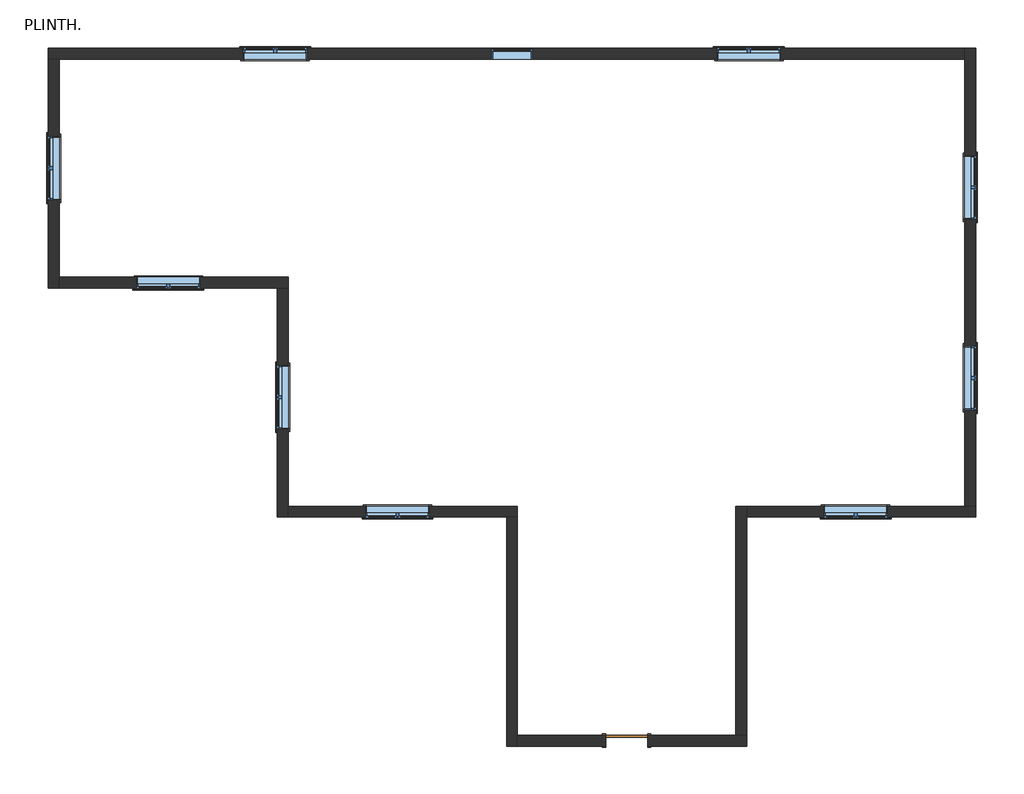
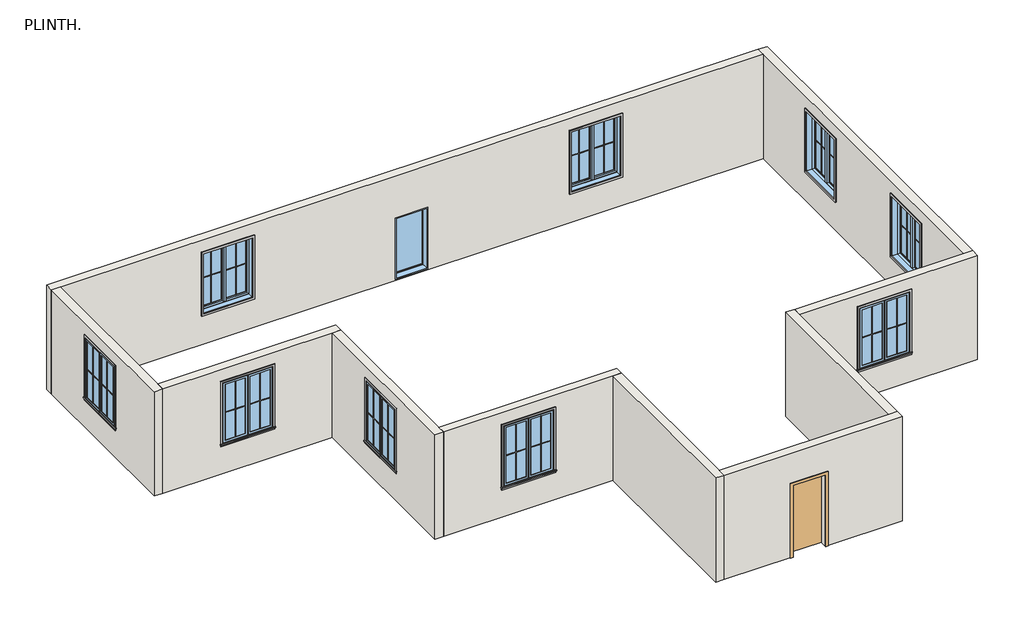
# One storey: 36 proxies, 10 walls, 10 windows, 1 door.
"""IFC4 building model written with IfcOpenShell, lengths in millimetres."""

import ifcopenshell
import ifcopenshell.guid

model = None  # the IFC model being written
_history = None  # IfcOwnerHistory: only IFC2X3 demands one
_inside = {}  # id of a spatial element -> (the spatial element, [elements in it])
_under = {}  # id of a project, library or spatial element -> (it, [spatial elements below it])
_declared = {}  # id of a project -> (the project, [libraries it declares])
_typed = {}  # id of a type object -> (the type object, [elements of that type])
_made_of = {}  # id of a material, layer set ... -> (it, [elements and type objects made of it])


def new_model(schema):
    """Start an empty IFC model of exactly this schema.

    Asked for "IFC4X3", IfcOpenShell would pick the latest addendum, in which some entities
    have other attributes; the version numbers below select the first issue.
    IFC2X3 requires an IfcOwnerHistory on every rooted entity: one is made here for all.
    """
    global model, _history
    if schema == "IFC4X3":
        model = ifcopenshell.file(schema_version=(4, 3, 0, 0))
    else:
        model = ifcopenshell.file(schema=schema)
    _inside.clear()
    _under.clear()
    _declared.clear()
    _typed.clear()
    _made_of.clear()
    _history = None
    if model.schema == "IFC2X3":
        org = make("IfcOrganization", Name="unknown")
        user = make(
            "IfcPersonAndOrganization",
            ThePerson=make("IfcPerson", FamilyName="unknown"),
            TheOrganization=org,
        )
        app = make(
            "IfcApplication",
            ApplicationDeveloper=org,
            Version="unknown",
            ApplicationFullName="unknown",
            ApplicationIdentifier="unknown",
        )
        _history = make(
            "IfcOwnerHistory",
            OwningUser=user,
            OwningApplication=app,
            ChangeAction="ADDED",
            CreationDate=0,
        )
    return model


def make(cls, **values):
    """One entity of the class cls with the attributes given. An attribute that is None is left unset."""
    return model.create_entity(
        cls, **{name: value for name, value in values.items() if value is not None}
    )


def rooted(cls, **values):
    """An entity with a GlobalId (a new one), such as an element, a storey or a relation."""
    return make(cls, GlobalId=ifcopenshell.guid.new(), OwnerHistory=_history, **values)


def si_unit(unit_type, name, prefix=None):
    """IfcSIUnit, for example si_unit("LENGTHUNIT", "METRE", prefix="MILLI")."""
    return make("IfcSIUnit", UnitType=unit_type, Prefix=prefix, Name=name)


def assignment(units):
    """IfcUnitAssignment: the units of a project."""
    return None if units is None else make("IfcUnitAssignment", Units=units)


def point(xyz):
    """IfcCartesianPoint."""
    return None if xyz is None else make("IfcCartesianPoint", Coordinates=xyz)


def direction(xyz):
    """IfcDirection."""
    return None if xyz is None else make("IfcDirection", DirectionRatios=xyz)


def frame(location, z_axis=None, x_axis=None):
    """IfcAxis2Placement3D, a coordinate frame: its origin and axes. An axis left out is left unset."""
    return make(
        "IfcAxis2Placement3D",
        Location=point(location),
        Axis=direction(z_axis),
        RefDirection=direction(x_axis),
    )


def origin():
    """The frame at (0, 0, 0) with its axes left unset."""
    return frame((0.0, 0.0, 0.0))


def origin_with_axes():
    """The frame at (0, 0, 0) with the z axis (0, 0, 1) and the x axis (1, 0, 0) written out."""
    return frame((0.0, 0.0, 0.0), z_axis=(0.0, 0.0, 1.0), x_axis=(1.0, 0.0, 0.0))


def place(relative_to, where):
    """IfcLocalPlacement: puts the frame where relative to a parent placement (None: the world)."""
    return make(
        "IfcLocalPlacement", PlacementRelTo=relative_to, RelativePlacement=where
    )


def context(
    kind, dimensions, precision=None, world=None, true_north=None, identifier=None
):
    """IfcGeometricRepresentationContext, for example the 3D "Model" context."""
    return make(
        "IfcGeometricRepresentationContext",
        ContextIdentifier=identifier,
        ContextType=kind,
        CoordinateSpaceDimension=dimensions,
        Precision=precision,
        WorldCoordinateSystem=world,
        TrueNorth=true_north,
    )


def project(units=None, contexts=None):
    """IfcProject with its units and contexts."""
    return rooted(
        "IfcProject",
        Name="project",
        RepresentationContexts=contexts,
        UnitsInContext=assignment(units),
    )


def spatial(cls, under=None, at=None, **own):
    """A site, building, storey or space (cls), placed at a placement, below another one or the project."""
    s = rooted(cls, ObjectPlacement=at, **own)
    if under is not None:
        _under.setdefault(under.id(), (under, []))[1].append(s)
    return s


def polyline(points):
    """IfcPolyline through the points."""
    return make("IfcPolyline", Points=[point(p) for p in points])


def outline(outer, holes=None, kind="AREA"):
    """IfcArbitraryClosedProfileDef: a profile drawn as a closed curve; with holes, ...WithVoids."""
    if holes is None:
        return make("IfcArbitraryClosedProfileDef", ProfileType=kind, OuterCurve=outer)
    return make(
        "IfcArbitraryProfileDefWithVoids",
        ProfileType=kind,
        OuterCurve=outer,
        InnerCurves=holes,
    )


def extrude(swept, where, along, depth):
    """IfcExtrudedAreaSolid: the profile swept, set in the frame where, extruded along a direction by depth."""
    return make(
        "IfcExtrudedAreaSolid",
        SweptArea=swept,
        Position=where,
        ExtrudedDirection=direction(along),
        Depth=depth,
    )


def faces_of(points, faces, orient=None, outer=None):
    """IfcFace entities. A face is a list of loops; a loop is a list of indices into points, from 0.

    orient and outer hold one flag for each loop. By default every Orientation is true, the
    first loop of a face is its IfcFaceOuterBound and the others are IfcFaceBound.
    """
    made = []
    for i, loops in enumerate(faces):
        bounds = []
        for j, loop in enumerate(loops):
            is_outer = j == 0 if outer is None else outer[i][j]
            bounds.append(
                make(
                    "IfcFaceOuterBound" if is_outer else "IfcFaceBound",
                    Bound=make("IfcPolyLoop", Polygon=[points[k] for k in loop]),
                    Orientation=True if orient is None else orient[i][j],
                )
            )
        made.append(make("IfcFace", Bounds=bounds))
    return made


def faceted_brep(points, faces, orient=None, outer=None, voids=None):
    """IfcFacetedBrep: a solid bounded by flat faces; with voids (closed shells), ...WithVoids."""
    shared = [point(p) for p in points]
    hull = make("IfcClosedShell", CfsFaces=faces_of(shared, faces, orient, outer))
    if voids is None:
        return make("IfcFacetedBrep", Outer=hull)
    return make(
        "IfcFacetedBrepWithVoids",
        Outer=hull,
        Voids=[
            make(cls, CfsFaces=faces_of(shared, fs, o, b)) for cls, fs, o, b in voids
        ],
    )


def shape(context_of_items, identifier, shape_type, items):
    """IfcShapeRepresentation: the items that make up one representation, for example the "Body"."""
    return make(
        "IfcShapeRepresentation",
        ContextOfItems=context_of_items,
        RepresentationIdentifier=identifier,
        RepresentationType=shape_type,
        Items=items,
    )


def source(mapping_origin, context_of_items, identifier, shape_type, items):
    """IfcRepresentationMap: a shape defined once, which mapped items show again and again."""
    return make(
        "IfcRepresentationMap",
        MappingOrigin=mapping_origin,
        MappedRepresentation=shape(context_of_items, identifier, shape_type, items),
    )


def transform(
    local_origin,
    x_axis=None,
    y_axis=None,
    z_axis=None,
    scale=None,
    scale2=None,
    scale3=None,
    uniform=True,
):
    """IfcCartesianTransformationOperator3D, or its non-uniform kind. x_axis, y_axis, z_axis: its Axis1, 2, 3."""
    if uniform:
        return make(
            "IfcCartesianTransformationOperator3D",
            Axis1=direction(x_axis),
            Axis2=direction(y_axis),
            LocalOrigin=point(local_origin),
            Scale=scale,
            Axis3=direction(z_axis),
        )
    return make(
        "IfcCartesianTransformationOperator3DnonUniform",
        Axis1=direction(x_axis),
        Axis2=direction(y_axis),
        LocalOrigin=point(local_origin),
        Scale=scale,
        Axis3=direction(z_axis),
        Scale2=scale2,
        Scale3=scale3,
    )


def mapped(mapping_source, mapping_target):
    """IfcMappedItem: shows the shape of a source again, moved by a transform."""
    return make(
        "IfcMappedItem", MappingSource=mapping_source, MappingTarget=mapping_target
    )


def made_of(thing, what):
    """Note that an element or type object is made of a material, layer set ...; save() writes the relation."""
    if what is not None:
        _made_of.setdefault(what.id(), (what, []))[1].append(thing)
    return thing


def element(
    cls,
    number,
    at=None,
    inside=None,
    cuts=None,
    type_object=None,
    material=None,
    context=None,
    identifier="Body",
    shape_type=None,
    held_by="IfcProductDefinitionShape",
    body=None,
    shapes=None,
    **own,
):
    """One element of the class cls, such as IfcWall. Its Tag is "e" and its number.

    at: its placement. inside: the storey or other place that contains it. cuts: it is an
    opening in that element (IfcRelVoidsElement). A single representation is given by context,
    identifier, shape_type and body (its items); several are given by shapes. held_by: the class
    of the entity that holds the representations. save() writes the other relations.
    """
    e = rooted(cls, Tag="e%d" % number, ObjectPlacement=at, **own)
    if body is not None:
        shapes = [shape(context, identifier, shape_type, body)]
    if shapes is not None:
        e.Representation = make(held_by, Representations=shapes)
    if inside is not None:
        _inside.setdefault(inside.id(), (inside, []))[1].append(e)
    if cuts is not None:
        rooted(
            "IfcRelVoidsElement", RelatingBuildingElement=cuts, RelatedOpeningElement=e
        )
    if type_object is not None:
        _typed.setdefault(type_object.id(), (type_object, []))[1].append(e)
    return made_of(e, material)


def aggregate(whole, parts):
    """IfcRelAggregates: a whole, such as a stair, and the parts it consists of."""
    return rooted("IfcRelAggregates", RelatingObject=whole, RelatedObjects=parts)


def save(model, path):
    """Write the relations noted so far, then the file.

    IfcRelAggregates (storeys below a building ...), IfcRelContainedInSpatialStructure (elements
    in a storey), IfcRelDefinesByType, IfcRelAssociatesMaterial and IfcRelDeclares: one each for
    every whole, place, type object, material and project.
    """
    for whole, parts in _under.values():
        aggregate(whole, parts)
    for where, things in _inside.values():
        rooted(
            "IfcRelContainedInSpatialStructure",
            RelatedElements=things,
            RelatingStructure=where,
        )
    for kind, things in _typed.values():
        rooted("IfcRelDefinesByType", RelatedObjects=things, RelatingType=kind)
    for what, things in _made_of.values():
        rooted("IfcRelAssociatesMaterial", RelatedObjects=things, RelatingMaterial=what)
    for by, libraries in _declared.values():
        rooted("IfcRelDeclares", RelatingContext=by, RelatedDefinitions=libraries)
    model.write(path)


def m_muntin_pattern_2x2_m_muntin_pattern_2x2_d2d4b859(model_context):
    return source(origin(), model_context, "Body", "SweptSolid", [
        extrude(outline(polyline([(836.5, -6.35), (836.5, -281.7375), (823.8, -281.7375), (823.8, -6.35), (0.0, -6.35), (0.0, 6.35), (823.8, 6.35), (823.8, 281.7375), (836.5, 281.7375), (836.5, 6.35), (1660.3, 6.35), (1660.3, -6.35), (836.5, -6.35)])), frame((0.0, 9.525, 0.0), z_axis=(0.0, 1.0, 0.0), x_axis=(0.0, 0.0, 1.0)), (0.0, 0.0, 1.0), 12.7),
        extrude(outline(polyline([(836.5, -6.35), (836.5, -281.7375), (823.8, -281.7375), (823.8, -6.35), (0.0, -6.35), (0.0, 6.35), (823.8, 6.35), (823.8, 281.7375), (836.5, 281.7375), (836.5, 6.35), (1660.3, 6.35), (1660.3, -6.35), (836.5, -6.35)])), frame((0.0, -22.225, 0.0), z_axis=(0.0, 1.0, 0.0), x_axis=(0.0, 0.0, 1.0)), (0.0, 0.0, 1.0), 12.7),
    ])


def m_muntin_pattern_2x2_m_muntin_pattern_2x2_f3921bb5(model_context):
    return source(origin(), model_context, "Body", "SweptSolid", [
        extrude(outline(polyline([(836.5, -6.35), (836.5, -281.7375), (823.8, -281.7375), (823.8, -6.35), (0.0, -6.35), (0.0, 6.35), (823.8, 6.35), (823.8, 281.7375), (836.5, 281.7375), (836.5, 6.35), (1660.3, 6.35), (1660.3, -6.35), (836.5, -6.35)])), frame((0.0, -22.225, 0.0), z_axis=(0.0, 1.0, 0.0), x_axis=(0.0, 0.0, 1.0)), (0.0, 0.0, 1.0), 12.7),
        extrude(outline(polyline([(836.5, -6.35), (836.5, -281.7375), (823.8, -281.7375), (823.8, -6.35), (0.0, -6.35), (0.0, 6.35), (823.8, 6.35), (823.8, 281.7375), (836.5, 281.7375), (836.5, 6.35), (1660.3, 6.35), (1660.3, -6.35), (836.5, -6.35)])), frame((0.0, 9.525, 0.0), z_axis=(0.0, 1.0, 0.0), x_axis=(0.0, 0.0, 1.0)), (0.0, 0.0, 1.0), 12.7),
    ])


def m_trim_window_exterior_flat_with_sill_136e302d(model_context):
    return source(origin(), model_context, "Body", "SweptSolid", [
        extrude(outline(polyline([(760.0, -1820.4323709), (760.0, -1880.4323709), (-760.0, -1880.4323709), (-760.0, -1820.4323709), (760.0, -1820.4323709)])), origin_with_axes(), (0.0, 0.0, 1.0), 19.05),
        extrude(outline(polyline([(-1830.0, 38.1), (-1802.4580645, 38.1), (-1800.0, 19.05), (-1800.0, 0.0), (-1820.4323709, 0.0), (-1820.4323709, 19.05), (-1830.0, 19.05), (-1830.0, 38.1)])), frame((-772.7, 0.0, 0.0), z_axis=(1.0, 0.0, 0.0), x_axis=(0.0, 1.0, 0.0)), (0.0, 0.0, 1.0), 1545.4),
        extrude(outline(polyline([(-760.0, 60.0), (760.0, 60.0), (760.0, -1800.0), (700.0, -1800.0), (700.0, 0.0), (-700.0, 0.0), (-700.0, -1800.0), (-760.0, -1800.0), (-760.0, 60.0)])), origin_with_axes(), (0.0, 0.0, 1.0), 19.05),
    ])


def m_trim_window_interior_flat_picture_frame_c6c50358(model_context):
    return source(origin(), model_context, "Body", "SweptSolid", [
        extrude(outline(polyline([(747.3, 47.3), (747.3, -1847.3), (-747.3, -1847.3), (-747.3, 47.3), (747.3, 47.3)]), holes=[polyline([(687.3, -12.7), (-687.3, -12.7), (-687.3, -1787.3), (687.3, -1787.3), (687.3, -12.7)])]), origin_with_axes(), (0.0, 0.0, 1.0), 30.0),
    ])


def m_single_flush_0915_x_2134mm_c020cfaa(model_context):
    return source(origin(), model_context, "Body", "SweptSolid", [
        extrude(outline(polyline([(2210.0, -533.5), (0.0, -533.5), (0.0, -457.5), (2134.0, -457.5), (2134.0, 457.5), (0.0, 457.5), (0.0, 533.5), (2210.0, 533.5), (2210.0, -533.5)])), frame((0.0, 120.0, 0.0), z_axis=(0.0, 1.0, 0.0), x_axis=(0.0, 0.0, 1.0)), (0.0, 0.0, 1.0), 25.0),
        extrude(outline(polyline([(2210.0, 533.5), (2210.0, -533.5), (0.0, -533.5), (0.0, -457.5), (2134.0, -457.5), (2134.0, 457.5), (0.0, 457.5), (0.0, 533.5), (2210.0, 533.5)])), frame((0.0, -145.0, 0.0), z_axis=(0.0, 1.0, 0.0), x_axis=(0.0, 0.0, 1.0)), (0.0, 0.0, 1.0), 25.0),
        extrude(outline(polyline([(457.5, 69.0), (-457.5, 69.0), (-457.5, 120.0), (457.5, 120.0), (457.5, 69.0)])), origin_with_axes(), (0.0, 0.0, 1.0), 2134.0),
    ])


def m_fixed_0915_x_1830mm_fa93d676(model_context):
    return source(origin(), model_context, "Body", "SweptSolid", [
        extrude(outline(polyline([(-394.5, 98.0), (394.5, 98.0), (394.5, 86.0), (-394.5, 86.0), (-394.5, 98.0)])), frame((0.0, 0.0, 368.0), z_axis=(0.0, 0.0, 1.0), x_axis=(1.0, 0.0, 0.0)), (0.0, 0.0, 1.0), 1704.0),
        extrude(outline(polyline([(2116.0, -438.5), (324.0, -438.5), (324.0, 438.5), (2116.0, 438.5), (2116.0, -438.5)]), holes=[polyline([(2072.0, -394.5), (2072.0, 394.5), (368.0, 394.5), (368.0, -394.5), (2072.0, -394.5)])]), frame((0.0, 70.0, 0.0), z_axis=(0.0, 1.0, 0.0), x_axis=(0.0, 0.0, 1.0)), (0.0, 0.0, 1.0), 44.0),
        extrude(outline(polyline([(2135.0, -457.5), (305.0, -457.5), (305.0, 457.5), (2135.0, 457.5), (2135.0, -457.5)]), holes=[polyline([(2116.0, -438.5), (2116.0, 438.5), (324.0, 438.5), (324.0, -438.5), (2116.0, -438.5)])]), frame((0.0, 70.0, 0.0), z_axis=(0.0, 1.0, 0.0), x_axis=(0.0, 0.0, 1.0)), (0.0, 0.0, 1.0), 63.0),
        extrude(outline(polyline([(2135.0, -457.5), (305.0, -457.5), (305.0, 457.5), (2135.0, 457.5), (2135.0, -457.5)]), holes=[polyline([(2103.0, -425.5), (2103.0, 425.5), (337.0, 425.5), (337.0, -425.5), (2103.0, -425.5)])]), frame((0.0, -107.0, 0.0), z_axis=(0.0, 1.0, 0.0), x_axis=(0.0, 0.0, 1.0)), (0.0, 0.0, 1.0), 177.0),
    ])


def m_window_casement_double_1400_x_1800mm_e3405f7f(model_context):
    return source(origin(), model_context, "Body", "SolidModel", [
        faceted_brep([(9.525, 139.05, 2687.3), (-9.525, 139.05, 2687.3), (-9.525, 88.25, 2687.3), (9.525, 88.25, 2687.3), (9.525, 139.05, 912.7), (9.525, 88.25, 912.7), (-9.525, 88.25, 912.7), (-9.525, 139.05, 912.7), (-9.525, 88.25, 931.75), (-9.525, 88.25, 2668.25), (-30.1625, 88.25, 931.75), (-30.1625, 88.25, 2668.25), (-30.1625, 24.75, 931.75), (-30.1625, 24.75, 2668.25), (30.1625, 24.75, 931.75), (30.1625, 24.75, 2668.25), (30.1625, 88.25, 931.75), (30.1625, 88.25, 2668.25), (9.525, 88.25, 931.75), (9.525, 88.25, 2668.25)], [[[0, 1, 2, 3]], [[4, 5, 6, 7]], [[1, 0, 4, 7]], [[2, 1, 7, 6, 8, 9]], [[9, 8, 10, 11]], [[11, 10, 12, 13]], [[13, 12, 14, 15]], [[15, 14, 16, 17]], [[17, 16, 18, 19]], [[0, 3, 19, 18, 5, 4]], [[18, 8, 6, 5]], [[9, 19, 3, 2]], [[8, 18, 16, 14, 12, 10]], [[19, 9, 11, 13, 15, 17]]]),
        extrude(outline(polyline([(-66.675, 120.0), (-66.675, 113.65), (-630.15, 113.65), (-630.15, 120.0), (-66.675, 120.0)])), frame((0.0, 0.0, 969.85), z_axis=(0.0, 0.0, 1.0), x_axis=(1.0, 0.0, 0.0)), (0.0, 0.0, 1.0), 1660.3),
        extrude(outline(polyline([(-630.15, 100.95), (-630.15, 107.3), (-66.675, 107.3), (-66.675, 100.95), (-630.15, 100.95)])), frame((0.0, 0.0, 969.85), z_axis=(0.0, 0.0, 1.0), x_axis=(1.0, 0.0, 0.0)), (0.0, 0.0, 1.0), 1660.3),
        extrude(outline(polyline([(630.15, 120.0), (630.15, 113.65), (66.675, 113.65), (66.675, 120.0), (630.15, 120.0)])), frame((0.0, 0.0, 969.85), z_axis=(0.0, 0.0, 1.0), x_axis=(1.0, 0.0, 0.0)), (0.0, 0.0, 1.0), 1660.3),
        extrude(outline(polyline([(66.675, 100.95), (66.675, 107.3), (630.15, 107.3), (630.15, 100.95), (66.675, 100.95)])), frame((0.0, 0.0, 969.85), z_axis=(0.0, 0.0, 1.0), x_axis=(1.0, 0.0, 0.0)), (0.0, 0.0, 1.0), 1660.3),
        extrude(outline(polyline([(2687.3, -687.3), (912.7, -687.3), (912.7, -9.525), (2687.3, -9.525), (2687.3, -687.3)]), holes=[polyline([(2630.15, -66.675), (969.85, -66.675), (969.85, -630.15), (2630.15, -630.15), (2630.15, -66.675)])]), frame((0.0, 88.25, 0.0), z_axis=(0.0, 1.0, 0.0), x_axis=(0.0, 0.0, 1.0)), (0.0, 0.0, 1.0), 44.45),
        extrude(outline(polyline([(912.7, 687.3), (2687.3, 687.3), (2687.3, 9.525), (912.7, 9.525), (912.7, 687.3)]), holes=[polyline([(969.85, 66.675), (2630.15, 66.675), (2630.15, 630.15), (969.85, 630.15), (969.85, 66.675)])]), frame((0.0, 88.25, 0.0), z_axis=(0.0, 1.0, 0.0), x_axis=(0.0, 0.0, 1.0)), (0.0, 0.0, 1.0), 44.45),
        extrude(outline(polyline([(2700.0, -700.0), (900.0, -700.0), (900.0, 700.0), (2700.0, 700.0), (2700.0, -700.0)]), holes=[polyline([(2680.95, 680.95), (919.05, 680.95), (919.05, -680.95), (2680.95, -680.95), (2680.95, 680.95)])]), frame((0.0, -120.0, 0.0), z_axis=(0.0, 1.0, 0.0), x_axis=(0.0, 0.0, 1.0)), (0.0, 0.0, 1.0), 144.75),
        faceted_brep([(668.25, 88.25, 2668.25), (668.25, 24.75, 2668.25), (-668.25, 24.75, 2668.25), (-668.25, 88.25, 2668.25), (687.3, 139.05, 2687.3), (687.3, 88.25, 2687.3), (-687.3, 88.25, 2687.3), (-687.3, 139.05, 2687.3), (700.0, 24.75, 2700.0), (700.0, 139.05, 2700.0), (-700.0, 139.05, 2700.0), (-700.0, 24.75, 2700.0), (-668.25, 24.75, 931.75), (-668.25, 88.25, 931.75), (-687.3, 88.25, 912.7), (-687.3, 139.05, 912.7), (-700.0, 139.05, 900.0), (-700.0, 24.75, 900.0), (668.25, 24.75, 931.75), (668.25, 88.25, 931.75), (687.3, 88.25, 912.7), (687.3, 139.05, 912.7), (700.0, 139.05, 900.0), (700.0, 24.75, 900.0)], [[[0, 1, 2, 3]], [[4, 5, 6, 7]], [[8, 9, 10, 11]], [[3, 2, 12, 13]], [[7, 6, 14, 15]], [[11, 10, 16, 17]], [[13, 12, 18, 19]], [[15, 14, 20, 21]], [[17, 16, 22, 23]], [[11, 17, 23, 8], [1, 18, 12, 2]], [[19, 18, 1, 0]], [[5, 20, 14, 6], [3, 13, 19, 0]], [[21, 20, 5, 4]], [[23, 22, 9, 8]], [[9, 22, 16, 10], [7, 15, 21, 4]]]),
    ])


model = new_model("IFC4")

# Units and contexts
model_context = context("Model", 3, world=origin())
ifc_project = project(units=[si_unit("LENGTHUNIT", "METRE", prefix="MILLI")], contexts=[model_context])

# Site, building, storey
site = spatial("IfcSite", under=ifc_project)
building = spatial("IfcBuilding", under=site)
storey = spatial("IfcBuildingStorey", under=building, Name="PLINTH.", Elevation=450.0)

# Proxies
placement = place(None, origin())
m_muntin_pattern_2x2_m_muntin_pattern_2x2_shape = m_muntin_pattern_2x2_m_muntin_pattern_2x2_d2d4b859(model_context)
element("IfcBuildingElementProxy", 1, Name="M_Muntin Pattern_2x2 : M_Muntin Pattern_2x2", ObjectType="M_Muntin Pattern_2x2 : M_Muntin Pattern_2x2", at=placement, inside=storey, context=model_context, shape_type="MappedRepresentation", body=[
    mapped(m_muntin_pattern_2x2_m_muntin_pattern_2x2_shape, transform((2989.733554, 14169.9094502, 1419.85), x_axis=(-1.0, 0.0, 0.0), y_axis=(0.0, -1.0, 0.0), z_axis=(0.0, 0.0, 1.0))),
])
element("IfcBuildingElementProxy", 2, Name="M_Muntin Pattern_2x2 : M_Muntin Pattern_2x2", ObjectType="M_Muntin Pattern_2x2 : M_Muntin Pattern_2x2", at=placement, inside=storey, context=model_context, shape_type="MappedRepresentation", body=[
    mapped(m_muntin_pattern_2x2_m_muntin_pattern_2x2_shape, transform((12989.733554, 14169.9094502, 1419.85), x_axis=(-1.0, 0.0, 0.0), y_axis=(0.0, -1.0, 0.0), z_axis=(0.0, 0.0, 1.0))),
])
element("IfcBuildingElementProxy", 3, Name="M_Muntin Pattern_2x2 : M_Muntin Pattern_2x2", ObjectType="M_Muntin Pattern_2x2 : M_Muntin Pattern_2x2", at=placement, inside=storey, context=model_context, shape_type="MappedRepresentation", body=[
    mapped(m_muntin_pattern_2x2_m_muntin_pattern_2x2_shape, transform((30.846054, 16431.9719502, 1419.85), x_axis=(0.0, 1.0, 0.0), y_axis=(-1.0, 0.0, 0.0), z_axis=(0.0, 0.0, 1.0))),
])
element("IfcBuildingElementProxy", 4, Name="M_Muntin Pattern_2x2 : M_Muntin Pattern_2x2", ObjectType="M_Muntin Pattern_2x2 : M_Muntin Pattern_2x2", at=placement, inside=storey, context=model_context, shape_type="MappedRepresentation", body=[
    mapped(m_muntin_pattern_2x2_m_muntin_pattern_2x2_shape, transform((-2010.266446, 19169.9094502, 1419.85), x_axis=(-1.0, 0.0, 0.0), y_axis=(0.0, -1.0, 0.0), z_axis=(0.0, 0.0, 1.0))),
])
element("IfcBuildingElementProxy", 5, Name="M_Muntin Pattern_2x2 : M_Muntin Pattern_2x2", ObjectType="M_Muntin Pattern_2x2 : M_Muntin Pattern_2x2", at=placement, inside=storey, context=model_context, shape_type="MappedRepresentation", body=[
    mapped(m_muntin_pattern_2x2_m_muntin_pattern_2x2_shape, transform((-4969.153946, 21431.9719502, 1419.85), x_axis=(0.0, 1.0, 0.0), y_axis=(-1.0, 0.0, 0.0), z_axis=(0.0, 0.0, 1.0))),
])
element("IfcBuildingElementProxy", 6, Name="M_Muntin Pattern_2x2 : M_Muntin Pattern_2x2", ObjectType="M_Muntin Pattern_2x2 : M_Muntin Pattern_2x2", at=placement, inside=storey, context=model_context, shape_type="MappedRepresentation", body=[
    mapped(m_muntin_pattern_2x2_m_muntin_pattern_2x2_shape, transform((-375.841446, 24390.8594502, 1419.85), x_axis=(1.0, 0.0, 0.0), y_axis=(0.0, 1.0, 0.0), z_axis=(0.0, 0.0, 1.0))),
])
element("IfcBuildingElementProxy", 7, Name="M_Muntin Pattern_2x2 : M_Muntin Pattern_2x2", ObjectType="M_Muntin Pattern_2x2 : M_Muntin Pattern_2x2", at=placement, inside=storey, context=model_context, shape_type="MappedRepresentation", body=[
    mapped(m_muntin_pattern_2x2_m_muntin_pattern_2x2_shape, transform((9961.658554, 24390.8594502, 1419.85), x_axis=(1.0, 0.0, 0.0), y_axis=(0.0, 1.0, 0.0), z_axis=(0.0, 0.0, 1.0))),
])
element("IfcBuildingElementProxy", 8, Name="M_Muntin Pattern_2x2 : M_Muntin Pattern_2x2", ObjectType="M_Muntin Pattern_2x2 : M_Muntin Pattern_2x2", at=placement, inside=storey, context=model_context, shape_type="MappedRepresentation", body=[
    mapped(m_muntin_pattern_2x2_m_muntin_pattern_2x2_shape, transform((15251.796054, 21708.7969502, 1419.85), x_axis=(0.0, -1.0, 0.0), y_axis=(1.0, 0.0, 0.0), z_axis=(0.0, 0.0, 1.0))),
])
element("IfcBuildingElementProxy", 9, Name="M_Muntin Pattern_2x2 : M_Muntin Pattern_2x2", ObjectType="M_Muntin Pattern_2x2 : M_Muntin Pattern_2x2", at=placement, inside=storey, context=model_context, shape_type="MappedRepresentation", body=[
    mapped(m_muntin_pattern_2x2_m_muntin_pattern_2x2_shape, transform((15251.796054, 17548.7969502, 1419.85), x_axis=(0.0, -1.0, 0.0), y_axis=(1.0, 0.0, 0.0), z_axis=(0.0, 0.0, 1.0))),
])
m_muntin_pattern_2x2_m_muntin_pattern_2x2_2_shape = m_muntin_pattern_2x2_m_muntin_pattern_2x2_f3921bb5(model_context)
element("IfcBuildingElementProxy", 10, Name="M_Muntin Pattern_2x2 : M_Muntin Pattern_2x2", ObjectType="M_Muntin Pattern_2x2 : M_Muntin Pattern_2x2", at=placement, inside=storey, context=model_context, shape_type="MappedRepresentation", body=[
    mapped(m_muntin_pattern_2x2_m_muntin_pattern_2x2_2_shape, transform((2292.908554, 14169.9094502, 1419.85), x_axis=(1.0, 0.0, 0.0), y_axis=(0.0, 1.0, 0.0), z_axis=(0.0, 0.0, 1.0))),
])
element("IfcBuildingElementProxy", 11, Name="M_Muntin Pattern_2x2 : M_Muntin Pattern_2x2", ObjectType="M_Muntin Pattern_2x2 : M_Muntin Pattern_2x2", at=placement, inside=storey, context=model_context, shape_type="MappedRepresentation", body=[
    mapped(m_muntin_pattern_2x2_m_muntin_pattern_2x2_2_shape, transform((12292.908554, 14169.9094502, 1419.85), x_axis=(1.0, 0.0, 0.0), y_axis=(0.0, 1.0, 0.0), z_axis=(0.0, 0.0, 1.0))),
])
element("IfcBuildingElementProxy", 12, Name="M_Muntin Pattern_2x2 : M_Muntin Pattern_2x2", ObjectType="M_Muntin Pattern_2x2 : M_Muntin Pattern_2x2", at=placement, inside=storey, context=model_context, shape_type="MappedRepresentation", body=[
    mapped(m_muntin_pattern_2x2_m_muntin_pattern_2x2_2_shape, transform((30.846054, 17128.7969502, 1419.85), x_axis=(0.0, -1.0, 0.0), y_axis=(1.0, 0.0, 0.0), z_axis=(0.0, 0.0, 1.0))),
])
element("IfcBuildingElementProxy", 13, Name="M_Muntin Pattern_2x2 : M_Muntin Pattern_2x2", ObjectType="M_Muntin Pattern_2x2 : M_Muntin Pattern_2x2", at=placement, inside=storey, context=model_context, shape_type="MappedRepresentation", body=[
    mapped(m_muntin_pattern_2x2_m_muntin_pattern_2x2_2_shape, transform((-2707.091446, 19169.9094502, 1419.85), x_axis=(1.0, 0.0, 0.0), y_axis=(0.0, 1.0, 0.0), z_axis=(0.0, 0.0, 1.0))),
])
element("IfcBuildingElementProxy", 14, Name="M_Muntin Pattern_2x2 : M_Muntin Pattern_2x2", ObjectType="M_Muntin Pattern_2x2 : M_Muntin Pattern_2x2", at=placement, inside=storey, context=model_context, shape_type="MappedRepresentation", body=[
    mapped(m_muntin_pattern_2x2_m_muntin_pattern_2x2_2_shape, transform((-4969.153946, 22128.7969502, 1419.85), x_axis=(0.0, -1.0, 0.0), y_axis=(1.0, 0.0, 0.0), z_axis=(0.0, 0.0, 1.0))),
])
element("IfcBuildingElementProxy", 15, Name="M_Muntin Pattern_2x2 : M_Muntin Pattern_2x2", ObjectType="M_Muntin Pattern_2x2 : M_Muntin Pattern_2x2", at=placement, inside=storey, context=model_context, shape_type="MappedRepresentation", body=[
    mapped(m_muntin_pattern_2x2_m_muntin_pattern_2x2_2_shape, transform((320.983554, 24390.8594502, 1419.85), x_axis=(-1.0, 0.0, 0.0), y_axis=(0.0, -1.0, 0.0), z_axis=(0.0, 0.0, 1.0))),
])
element("IfcBuildingElementProxy", 16, Name="M_Muntin Pattern_2x2 : M_Muntin Pattern_2x2", ObjectType="M_Muntin Pattern_2x2 : M_Muntin Pattern_2x2", at=placement, inside=storey, context=model_context, shape_type="MappedRepresentation", body=[
    mapped(m_muntin_pattern_2x2_m_muntin_pattern_2x2_2_shape, transform((10658.483554, 24390.8594502, 1419.85), x_axis=(-1.0, 0.0, 0.0), y_axis=(0.0, -1.0, 0.0), z_axis=(0.0, 0.0, 1.0))),
])
element("IfcBuildingElementProxy", 17, Name="M_Muntin Pattern_2x2 : M_Muntin Pattern_2x2", ObjectType="M_Muntin Pattern_2x2 : M_Muntin Pattern_2x2", at=placement, inside=storey, context=model_context, shape_type="MappedRepresentation", body=[
    mapped(m_muntin_pattern_2x2_m_muntin_pattern_2x2_2_shape, transform((15251.796054, 21011.9719502, 1419.85), x_axis=(0.0, 1.0, 0.0), y_axis=(-1.0, 0.0, 0.0), z_axis=(0.0, 0.0, 1.0))),
])
element("IfcBuildingElementProxy", 18, Name="M_Muntin Pattern_2x2 : M_Muntin Pattern_2x2", ObjectType="M_Muntin Pattern_2x2 : M_Muntin Pattern_2x2", at=placement, inside=storey, context=model_context, shape_type="MappedRepresentation", body=[
    mapped(m_muntin_pattern_2x2_m_muntin_pattern_2x2_2_shape, transform((15251.796054, 16851.9719502, 1419.85), x_axis=(0.0, 1.0, 0.0), y_axis=(-1.0, 0.0, 0.0), z_axis=(0.0, 0.0, 1.0))),
])
m_trim_window_exterior_flat_with_sill_shape = m_trim_window_exterior_flat_with_sill_136e302d(model_context)
element("IfcBuildingElementProxy", 19, Name="M_Trim-Window-Exterior-Flat : with Sill", ObjectType="M_Trim-Window-Exterior-Flat : with Sill", at=placement, inside=storey, context=model_context, shape_type="MappedRepresentation", body=[
    mapped(m_trim_window_exterior_flat_with_sill_shape, transform((2641.321054, 14160.3844502, 3150.0), x_axis=(1.0, 0.0, 0.0), y_axis=(0.0, 0.0, 1.0), z_axis=(0.0, -1.0, 0.0))),
])
element("IfcBuildingElementProxy", 20, Name="M_Trim-Window-Exterior-Flat : with Sill", ObjectType="M_Trim-Window-Exterior-Flat : with Sill", at=placement, inside=storey, context=model_context, shape_type="MappedRepresentation", body=[
    mapped(m_trim_window_exterior_flat_with_sill_shape, transform((12641.321054, 14160.3844502, 3150.0), x_axis=(1.0, 0.0, 0.0), y_axis=(0.0, 0.0, 1.0), z_axis=(0.0, -1.0, 0.0))),
])
element("IfcBuildingElementProxy", 21, Name="M_Trim-Window-Exterior-Flat : with Sill", ObjectType="M_Trim-Window-Exterior-Flat : with Sill", at=placement, inside=storey, context=model_context, shape_type="MappedRepresentation", body=[
    mapped(m_trim_window_exterior_flat_with_sill_shape, transform((21.321054, 16780.3844502, 3150.0), x_axis=(0.0, -1.0, 0.0), y_axis=(0.0, 0.0, 1.0), z_axis=(-1.0, 0.0, 0.0))),
])
element("IfcBuildingElementProxy", 22, Name="M_Trim-Window-Exterior-Flat : with Sill", ObjectType="M_Trim-Window-Exterior-Flat : with Sill", at=placement, inside=storey, context=model_context, shape_type="MappedRepresentation", body=[
    mapped(m_trim_window_exterior_flat_with_sill_shape, transform((-2358.678946, 19160.3844502, 3150.0), x_axis=(1.0, 0.0, 0.0), y_axis=(0.0, 0.0, 1.0), z_axis=(0.0, -1.0, 0.0))),
])
element("IfcBuildingElementProxy", 23, Name="M_Trim-Window-Exterior-Flat : with Sill", ObjectType="M_Trim-Window-Exterior-Flat : with Sill", at=placement, inside=storey, context=model_context, shape_type="MappedRepresentation", body=[
    mapped(m_trim_window_exterior_flat_with_sill_shape, transform((-4978.678946, 21780.3844502, 3150.0), x_axis=(0.0, -1.0, 0.0), y_axis=(0.0, 0.0, 1.0), z_axis=(-1.0, 0.0, 0.0))),
])
element("IfcBuildingElementProxy", 24, Name="M_Trim-Window-Exterior-Flat : with Sill", ObjectType="M_Trim-Window-Exterior-Flat : with Sill", at=placement, inside=storey, context=model_context, shape_type="MappedRepresentation", body=[
    mapped(m_trim_window_exterior_flat_with_sill_shape, transform((-27.428946, 24400.3844502, 3150.0), x_axis=(-1.0, 0.0, 0.0), y_axis=(0.0, 0.0, 1.0), z_axis=(0.0, 1.0, 0.0))),
])
element("IfcBuildingElementProxy", 25, Name="M_Trim-Window-Exterior-Flat : with Sill", ObjectType="M_Trim-Window-Exterior-Flat : with Sill", at=placement, inside=storey, context=model_context, shape_type="MappedRepresentation", body=[
    mapped(m_trim_window_exterior_flat_with_sill_shape, transform((10310.071054, 24400.3844502, 3150.0), x_axis=(-1.0, 0.0, 0.0), y_axis=(0.0, 0.0, 1.0), z_axis=(0.0, 1.0, 0.0))),
])
element("IfcBuildingElementProxy", 26, Name="M_Trim-Window-Exterior-Flat : with Sill", ObjectType="M_Trim-Window-Exterior-Flat : with Sill", at=placement, inside=storey, context=model_context, shape_type="MappedRepresentation", body=[
    mapped(m_trim_window_exterior_flat_with_sill_shape, transform((15261.321054, 21360.3844502, 3150.0), x_axis=(0.0, 1.0, 0.0), y_axis=(0.0, 0.0, 1.0), z_axis=(1.0, 0.0, 0.0))),
])
element("IfcBuildingElementProxy", 27, Name="M_Trim-Window-Exterior-Flat : with Sill", ObjectType="M_Trim-Window-Exterior-Flat : with Sill", at=placement, inside=storey, context=model_context, shape_type="MappedRepresentation", body=[
    mapped(m_trim_window_exterior_flat_with_sill_shape, transform((15261.321054, 17200.3844502, 3150.0), x_axis=(0.0, 1.0, 0.0), y_axis=(0.0, 0.0, 1.0), z_axis=(1.0, 0.0, 0.0))),
])
m_trim_window_interior_flat_picture_frame_shape = m_trim_window_interior_flat_picture_frame_c6c50358(model_context)
element("IfcBuildingElementProxy", 28, Name="M_Trim-Window-Interior-Flat : Picture Frame", ObjectType="M_Trim-Window-Interior-Flat : Picture Frame", at=placement, inside=storey, context=model_context, shape_type="MappedRepresentation", body=[
    mapped(m_trim_window_interior_flat_picture_frame_shape, transform((2641.321054, 14400.3844502, 3150.0), x_axis=(-1.0, 0.0, 0.0), y_axis=(0.0, 0.0, 1.0), z_axis=(0.0, 1.0, 0.0))),
])
element("IfcBuildingElementProxy", 29, Name="M_Trim-Window-Interior-Flat : Picture Frame", ObjectType="M_Trim-Window-Interior-Flat : Picture Frame", at=placement, inside=storey, context=model_context, shape_type="MappedRepresentation", body=[
    mapped(m_trim_window_interior_flat_picture_frame_shape, transform((12641.321054, 14400.3844502, 3150.0), x_axis=(-1.0, 0.0, 0.0), y_axis=(0.0, 0.0, 1.0), z_axis=(0.0, 1.0, 0.0))),
])
element("IfcBuildingElementProxy", 30, Name="M_Trim-Window-Interior-Flat : Picture Frame", ObjectType="M_Trim-Window-Interior-Flat : Picture Frame", at=placement, inside=storey, context=model_context, shape_type="MappedRepresentation", body=[
    mapped(m_trim_window_interior_flat_picture_frame_shape, transform((261.321054, 16780.3844502, 3150.0), x_axis=(0.0, 1.0, 0.0), y_axis=(0.0, 0.0, 1.0), z_axis=(1.0, 0.0, 0.0))),
])
element("IfcBuildingElementProxy", 31, Name="M_Trim-Window-Interior-Flat : Picture Frame", ObjectType="M_Trim-Window-Interior-Flat : Picture Frame", at=placement, inside=storey, context=model_context, shape_type="MappedRepresentation", body=[
    mapped(m_trim_window_interior_flat_picture_frame_shape, transform((-2358.678946, 19400.3844502, 3150.0), x_axis=(-1.0, 0.0, 0.0), y_axis=(0.0, 0.0, 1.0), z_axis=(0.0, 1.0, 0.0))),
])
element("IfcBuildingElementProxy", 32, Name="M_Trim-Window-Interior-Flat : Picture Frame", ObjectType="M_Trim-Window-Interior-Flat : Picture Frame", at=placement, inside=storey, context=model_context, shape_type="MappedRepresentation", body=[
    mapped(m_trim_window_interior_flat_picture_frame_shape, transform((-4738.678946, 21780.3844502, 3150.0), x_axis=(0.0, 1.0, 0.0), y_axis=(0.0, 0.0, 1.0), z_axis=(1.0, 0.0, 0.0))),
])
element("IfcBuildingElementProxy", 33, Name="M_Trim-Window-Interior-Flat : Picture Frame", ObjectType="M_Trim-Window-Interior-Flat : Picture Frame", at=placement, inside=storey, context=model_context, shape_type="MappedRepresentation", body=[
    mapped(m_trim_window_interior_flat_picture_frame_shape, transform((-27.428946, 24160.3844502, 3150.0), x_axis=(1.0, 0.0, 0.0), y_axis=(0.0, 0.0, 1.0), z_axis=(0.0, -1.0, 0.0))),
])
element("IfcBuildingElementProxy", 34, Name="M_Trim-Window-Interior-Flat : Picture Frame", ObjectType="M_Trim-Window-Interior-Flat : Picture Frame", at=placement, inside=storey, context=model_context, shape_type="MappedRepresentation", body=[
    mapped(m_trim_window_interior_flat_picture_frame_shape, transform((10310.071054, 24160.3844502, 3150.0), x_axis=(1.0, 0.0, 0.0), y_axis=(0.0, 0.0, 1.0), z_axis=(0.0, -1.0, 0.0))),
])
element("IfcBuildingElementProxy", 35, Name="M_Trim-Window-Interior-Flat : Picture Frame", ObjectType="M_Trim-Window-Interior-Flat : Picture Frame", at=placement, inside=storey, context=model_context, shape_type="MappedRepresentation", body=[
    mapped(m_trim_window_interior_flat_picture_frame_shape, transform((15021.321054, 21360.3844502, 3150.0), x_axis=(0.0, -1.0, 0.0), y_axis=(0.0, 0.0, 1.0), z_axis=(-1.0, 0.0, 0.0))),
])
element("IfcBuildingElementProxy", 36, Name="M_Trim-Window-Interior-Flat : Picture Frame", ObjectType="M_Trim-Window-Interior-Flat : Picture Frame", at=placement, inside=storey, context=model_context, shape_type="MappedRepresentation", body=[
    mapped(m_trim_window_interior_flat_picture_frame_shape, transform((15021.321054, 17200.3844502, 3150.0), x_axis=(0.0, -1.0, 0.0), y_axis=(0.0, 0.0, 1.0), z_axis=(-1.0, 0.0, 0.0))),
])

# Door
m_single_flush_0915_x_2134mm_shape = m_single_flush_0915_x_2134mm_c020cfaa(model_context)
element("IfcDoor", 37, ObjectType="M_Single-Flush : 0915 x 2134mm", at=placement, inside=storey, context=model_context, shape_type="MappedRepresentation", body=[
    mapped(m_single_flush_0915_x_2134mm_shape, transform((7641.321054, 9280.3844502, 450.0), x_axis=(1.0, 0.0, 0.0), y_axis=(0.0, 1.0, 0.0), z_axis=(0.0, 0.0, 1.0))),
])

# Walls
element("IfcWall", 38, ObjectType="WALL24", at=placement, inside=storey, context=model_context, shape_type="Brep", body=[
    faceted_brep([(15021.321054, 24400.3844502, 450.0), (-4978.678946, 24400.3844502, 450.0), (-4978.678946, 24400.3844502, 3550.0), (15021.321054, 24400.3844502, 3550.0), (4683.821054, 24400.3844502, 470.0), (5598.821054, 24400.3844502, 470.0), (5598.821054, 24400.3844502, 2300.0), (4683.821054, 24400.3844502, 2300.0), (672.571054, 24400.3844502, 3150.0), (-727.428946, 24400.3844502, 3150.0), (-727.428946, 24400.3844502, 1350.0), (672.571054, 24400.3844502, 1350.0), (11010.071054, 24400.3844502, 3150.0), (9610.071054, 24400.3844502, 3150.0), (9610.071054, 24400.3844502, 1350.0), (11010.071054, 24400.3844502, 1350.0), (15021.321054, 24160.3844502, 450.0), (15021.321054, 24160.3844502, 3550.0), (-4738.678946, 24160.3844502, 3550.0), (-4978.678946, 24160.3844502, 3550.0), (-4978.678946, 24160.3844502, 450.0), (-4738.678946, 24160.3844502, 450.0), (4683.821054, 24160.3844502, 470.0), (4683.821054, 24160.3844502, 2300.0), (5598.821054, 24160.3844502, 2300.0), (5598.821054, 24160.3844502, 470.0), (672.571054, 24160.3844502, 3150.0), (672.571054, 24160.3844502, 1350.0), (-727.428946, 24160.3844502, 1350.0), (-727.428946, 24160.3844502, 3150.0), (11010.071054, 24160.3844502, 3150.0), (11010.071054, 24160.3844502, 1350.0), (9610.071054, 24160.3844502, 1350.0), (9610.071054, 24160.3844502, 3150.0)], [[[0, 1, 2, 3], [4, 5, 6, 7], [8, 9, 10, 11], [12, 13, 14, 15]], [[16, 17, 18, 19, 20, 21], [22, 23, 24, 25], [26, 27, 28, 29], [30, 31, 32, 33]], [[1, 0, 16, 21, 20]], [[3, 2, 19, 18, 17]], [[2, 1, 20, 19]], [[0, 3, 17, 16]], [[23, 22, 4, 7]], [[24, 23, 7, 6]], [[25, 24, 6, 5]], [[22, 25, 5, 4]], [[27, 26, 8, 11]], [[28, 27, 11, 10]], [[29, 28, 10, 9]], [[26, 29, 9, 8]], [[31, 30, 12, 15]], [[32, 31, 15, 14]], [[33, 32, 14, 13]], [[30, 33, 13, 12]]]),
])
element("IfcWall", 39, ObjectType="WALL24", at=placement, inside=storey, context=model_context, shape_type="Brep", body=[
    faceted_brep([(-4978.678946, 24160.3844502, 450.0), (-4978.678946, 19160.3844502, 450.0), (-4978.678946, 19160.3844502, 3550.0), (-4978.678946, 24160.3844502, 3550.0), (-4978.678946, 22480.3844502, 3150.0), (-4978.678946, 21080.3844502, 3150.0), (-4978.678946, 21080.3844502, 1350.0), (-4978.678946, 22480.3844502, 1350.0), (-4738.678946, 24160.3844502, 450.0), (-4738.678946, 24160.3844502, 3550.0), (-4738.678946, 19400.3844502, 3550.0), (-4738.678946, 19160.3844502, 3550.0), (-4738.678946, 19160.3844502, 450.0), (-4738.678946, 19400.3844502, 450.0), (-4738.678946, 22480.3844502, 3150.0), (-4738.678946, 22480.3844502, 1350.0), (-4738.678946, 21080.3844502, 1350.0), (-4738.678946, 21080.3844502, 3150.0)], [[[0, 1, 2, 3], [4, 5, 6, 7]], [[8, 9, 10, 11, 12, 13], [14, 15, 16, 17]], [[1, 0, 8, 13, 12]], [[3, 2, 11, 10, 9]], [[0, 3, 9, 8]], [[2, 1, 12, 11]], [[15, 14, 4, 7]], [[16, 15, 7, 6]], [[17, 16, 6, 5]], [[14, 17, 5, 4]]]),
])
element("IfcWall", 40, ObjectType="WALL24", at=placement, inside=storey, context=model_context, shape_type="Brep", body=[
    faceted_brep([(-4738.678946, 19160.3844502, 450.0), (21.321054, 19160.3844502, 450.0), (261.321054, 19160.3844502, 450.0), (261.321054, 19160.3844502, 3550.0), (21.321054, 19160.3844502, 3550.0), (-4738.678946, 19160.3844502, 3550.0), (-3058.678946, 19160.3844502, 3150.0), (-1658.678946, 19160.3844502, 3150.0), (-1658.678946, 19160.3844502, 1350.0), (-3058.678946, 19160.3844502, 1350.0), (-4738.678946, 19400.3844502, 450.0), (-4738.678946, 19400.3844502, 3550.0), (261.321054, 19400.3844502, 3550.0), (261.321054, 19400.3844502, 450.0), (-3058.678946, 19400.3844502, 3150.0), (-3058.678946, 19400.3844502, 1350.0), (-1658.678946, 19400.3844502, 1350.0), (-1658.678946, 19400.3844502, 3150.0)], [[[0, 1, 2, 3, 4, 5], [6, 7, 8, 9]], [[10, 11, 12, 13], [14, 15, 16, 17]], [[2, 1, 0, 10, 13]], [[5, 4, 3, 12, 11]], [[0, 5, 11, 10]], [[3, 2, 13, 12]], [[15, 14, 6, 9]], [[16, 15, 9, 8]], [[17, 16, 8, 7]], [[14, 17, 7, 6]]]),
])
element("IfcWall", 41, ObjectType="WALL24", at=placement, inside=storey, context=model_context, shape_type="Brep", body=[
    faceted_brep([(21.321054, 19160.3844502, 450.0), (21.321054, 14160.3844502, 450.0), (21.321054, 14160.3844502, 3550.0), (21.321054, 19160.3844502, 3550.0), (21.321054, 17480.3844502, 3150.0), (21.321054, 16080.3844502, 3150.0), (21.321054, 16080.3844502, 1350.0), (21.321054, 17480.3844502, 1350.0), (261.321054, 19160.3844502, 450.0), (261.321054, 19160.3844502, 3550.0), (261.321054, 14400.3844502, 3550.0), (261.321054, 14160.3844502, 3550.0), (261.321054, 14160.3844502, 450.0), (261.321054, 14400.3844502, 450.0), (261.321054, 17480.3844502, 3150.0), (261.321054, 17480.3844502, 1350.0), (261.321054, 16080.3844502, 1350.0), (261.321054, 16080.3844502, 3150.0)], [[[0, 1, 2, 3], [4, 5, 6, 7]], [[8, 9, 10, 11, 12, 13], [14, 15, 16, 17]], [[1, 0, 8, 13, 12]], [[3, 2, 11, 10, 9]], [[0, 3, 9, 8]], [[2, 1, 12, 11]], [[15, 14, 4, 7]], [[16, 15, 7, 6]], [[17, 16, 6, 5]], [[14, 17, 5, 4]]]),
])
element("IfcWall", 42, ObjectType="WALL24", at=placement, inside=storey, context=model_context, shape_type="Brep", body=[
    faceted_brep([(261.321054, 14160.3844502, 450.0), (5021.321054, 14160.3844502, 450.0), (5261.321054, 14160.3844502, 450.0), (5261.321054, 14160.3844502, 3550.0), (5021.321054, 14160.3844502, 3550.0), (261.321054, 14160.3844502, 3550.0), (1941.321054, 14160.3844502, 3150.0), (3341.321054, 14160.3844502, 3150.0), (3341.321054, 14160.3844502, 1350.0), (1941.321054, 14160.3844502, 1350.0), (261.321054, 14400.3844502, 450.0), (261.321054, 14400.3844502, 3550.0), (5261.321054, 14400.3844502, 3550.0), (5261.321054, 14400.3844502, 450.0), (1941.321054, 14400.3844502, 3150.0), (1941.321054, 14400.3844502, 1350.0), (3341.321054, 14400.3844502, 1350.0), (3341.321054, 14400.3844502, 3150.0)], [[[0, 1, 2, 3, 4, 5], [6, 7, 8, 9]], [[10, 11, 12, 13], [14, 15, 16, 17]], [[2, 1, 0, 10, 13]], [[5, 4, 3, 12, 11]], [[0, 5, 11, 10]], [[3, 2, 13, 12]], [[15, 14, 6, 9]], [[16, 15, 9, 8]], [[17, 16, 8, 7]], [[14, 17, 7, 6]]]),
])
element("IfcWall", 43, ObjectType="WALL24", at=placement, inside=storey, context=model_context, shape_type="Brep", body=[
    faceted_brep([(5021.321054, 14160.3844502, 450.0), (5021.321054, 9160.3844502, 450.0), (5021.321054, 9160.3844502, 3550.0), (5021.321054, 14160.3844502, 3550.0), (5261.321054, 14160.3844502, 450.0), (5261.321054, 14160.3844502, 3550.0), (5261.321054, 9400.3844502, 3550.0), (5261.321054, 9160.3844502, 3550.0), (5261.321054, 9160.3844502, 450.0), (5261.321054, 9400.3844502, 450.0)], [[[0, 1, 2, 3]], [[4, 5, 6, 7, 8, 9]], [[1, 0, 4, 9, 8]], [[3, 2, 7, 6, 5]], [[0, 3, 5, 4]], [[2, 1, 8, 7]]]),
])
element("IfcWall", 44, ObjectType="WALL24", at=placement, inside=storey, context=model_context, shape_type="Brep", body=[
    faceted_brep([(8098.821054, 9160.3844502, 2584.0), (8098.821054, 9160.3844502, 450.0), (10261.321054, 9160.3844502, 450.0), (10261.321054, 9160.3844502, 3550.0), (5261.321054, 9160.3844502, 3550.0), (5261.321054, 9160.3844502, 450.0), (7183.821054, 9160.3844502, 450.0), (7183.821054, 9160.3844502, 2584.0), (10261.321054, 9400.3844502, 450.0), (10021.321054, 9400.3844502, 450.0), (8098.821054, 9400.3844502, 450.0), (8098.821054, 9400.3844502, 2584.0), (7183.821054, 9400.3844502, 2584.0), (7183.821054, 9400.3844502, 450.0), (5261.321054, 9400.3844502, 450.0), (5261.321054, 9400.3844502, 3550.0), (10021.321054, 9400.3844502, 3550.0), (10261.321054, 9400.3844502, 3550.0)], [[[0, 1, 2, 3, 4, 5, 6, 7]], [[8, 9, 10, 11, 12, 13, 14, 15, 16, 17]], [[6, 5, 14, 13]], [[2, 1, 10, 9, 8]], [[4, 3, 17, 16, 15]], [[5, 4, 15, 14]], [[3, 2, 8, 17]], [[11, 10, 1, 0]], [[12, 11, 0, 7]], [[13, 12, 7, 6]]]),
])
element("IfcWall", 45, ObjectType="WALL24", at=placement, inside=storey, context=model_context, shape_type="Brep", body=[
    faceted_brep([(10261.321054, 9400.3844502, 450.0), (10261.321054, 14160.3844502, 450.0), (10261.321054, 14400.3844502, 450.0), (10261.321054, 14400.3844502, 3550.0), (10261.321054, 14160.3844502, 3550.0), (10261.321054, 9400.3844502, 3550.0), (10021.321054, 9400.3844502, 450.0), (10021.321054, 9400.3844502, 3550.0), (10021.321054, 14400.3844502, 3550.0), (10021.321054, 14400.3844502, 450.0)], [[[0, 1, 2, 3, 4, 5]], [[6, 7, 8, 9]], [[2, 1, 0, 6, 9]], [[5, 4, 3, 8, 7]], [[0, 5, 7, 6]], [[3, 2, 9, 8]]]),
])
element("IfcWall", 46, ObjectType="WALL24", at=placement, inside=storey, context=model_context, shape_type="Brep", body=[
    faceted_brep([(10261.321054, 14160.3844502, 450.0), (15261.321054, 14160.3844502, 450.0), (15261.321054, 14160.3844502, 3550.0), (10261.321054, 14160.3844502, 3550.0), (11941.321054, 14160.3844502, 3150.0), (13341.321054, 14160.3844502, 3150.0), (13341.321054, 14160.3844502, 1350.0), (11941.321054, 14160.3844502, 1350.0), (10261.321054, 14400.3844502, 450.0), (10261.321054, 14400.3844502, 3550.0), (15021.321054, 14400.3844502, 3550.0), (15261.321054, 14400.3844502, 3550.0), (15261.321054, 14400.3844502, 450.0), (15021.321054, 14400.3844502, 450.0), (11941.321054, 14400.3844502, 3150.0), (11941.321054, 14400.3844502, 1350.0), (13341.321054, 14400.3844502, 1350.0), (13341.321054, 14400.3844502, 3150.0)], [[[0, 1, 2, 3], [4, 5, 6, 7]], [[8, 9, 10, 11, 12, 13], [14, 15, 16, 17]], [[1, 0, 8, 13, 12]], [[3, 2, 11, 10, 9]], [[0, 3, 9, 8]], [[2, 1, 12, 11]], [[15, 14, 4, 7]], [[16, 15, 7, 6]], [[17, 16, 6, 5]], [[14, 17, 5, 4]]]),
])
element("IfcWall", 47, ObjectType="WALL24", at=placement, inside=storey, context=model_context, shape_type="Brep", body=[
    faceted_brep([(15261.321054, 14400.3844502, 450.0), (15261.321054, 24400.3844502, 450.0), (15261.321054, 24400.3844502, 3550.0), (15261.321054, 14400.3844502, 3550.0), (15261.321054, 20660.3844502, 3150.0), (15261.321054, 22060.3844502, 3150.0), (15261.321054, 22060.3844502, 1350.0), (15261.321054, 20660.3844502, 1350.0), (15261.321054, 16500.3844502, 3150.0), (15261.321054, 17900.3844502, 3150.0), (15261.321054, 17900.3844502, 1350.0), (15261.321054, 16500.3844502, 1350.0), (15021.321054, 14400.3844502, 450.0), (15021.321054, 14400.3844502, 3550.0), (15021.321054, 24160.3844502, 3550.0), (15021.321054, 24400.3844502, 3550.0), (15021.321054, 24400.3844502, 450.0), (15021.321054, 24160.3844502, 450.0), (15021.321054, 20660.3844502, 3150.0), (15021.321054, 20660.3844502, 1350.0), (15021.321054, 22060.3844502, 1350.0), (15021.321054, 22060.3844502, 3150.0), (15021.321054, 16500.3844502, 3150.0), (15021.321054, 16500.3844502, 1350.0), (15021.321054, 17900.3844502, 1350.0), (15021.321054, 17900.3844502, 3150.0)], [[[0, 1, 2, 3], [4, 5, 6, 7], [8, 9, 10, 11]], [[12, 13, 14, 15, 16, 17], [18, 19, 20, 21], [22, 23, 24, 25]], [[1, 0, 12, 17, 16]], [[3, 2, 15, 14, 13]], [[0, 3, 13, 12]], [[2, 1, 16, 15]], [[19, 18, 4, 7]], [[20, 19, 7, 6]], [[21, 20, 6, 5]], [[18, 21, 5, 4]], [[23, 22, 8, 11]], [[24, 23, 11, 10]], [[25, 24, 10, 9]], [[22, 25, 9, 8]]]),
])

# Windows
m_fixed_0915_x_1830mm_shape = m_fixed_0915_x_1830mm_fa93d676(model_context)
element("IfcWindow", 48, ObjectType="M_Fixed : 0915 x 1830mm", at=placement, inside=storey, context=model_context, shape_type="MappedRepresentation", body=[
    mapped(m_fixed_0915_x_1830mm_shape, transform((5141.321054, 24267.3844502, 165.0), x_axis=(1.0, 0.0, 0.0), y_axis=(0.0, 1.0, 0.0), z_axis=(0.0, 0.0, 1.0))),
])
m_window_casement_double_1400_x_1800mm_shape = m_window_casement_double_1400_x_1800mm_e3405f7f(model_context)
element("IfcWindow", 49, ObjectType="M_Window-Casement-Double : 1400 x 1800mm", at=placement, inside=storey, context=model_context, shape_type="MappedRepresentation", body=[
    mapped(m_window_casement_double_1400_x_1800mm_shape, transform((2641.321054, 14280.3844502, 450.0), x_axis=(-1.0, 0.0, 0.0), y_axis=(0.0, -1.0, 0.0), z_axis=(0.0, 0.0, 1.0))),
])
element("IfcWindow", 50, ObjectType="M_Window-Casement-Double : 1400 x 1800mm", at=placement, inside=storey, context=model_context, shape_type="MappedRepresentation", body=[
    mapped(m_window_casement_double_1400_x_1800mm_shape, transform((12641.321054, 14280.3844502, 450.0), x_axis=(-1.0, 0.0, 0.0), y_axis=(0.0, -1.0, 0.0), z_axis=(0.0, 0.0, 1.0))),
])
element("IfcWindow", 51, ObjectType="M_Window-Casement-Double : 1400 x 1800mm", at=placement, inside=storey, context=model_context, shape_type="MappedRepresentation", body=[
    mapped(m_window_casement_double_1400_x_1800mm_shape, transform((141.321054, 16780.3844502, 450.0), x_axis=(0.0, 1.0, 0.0), y_axis=(-1.0, 0.0, 0.0), z_axis=(0.0, 0.0, 1.0))),
])
element("IfcWindow", 52, ObjectType="M_Window-Casement-Double : 1400 x 1800mm", at=placement, inside=storey, context=model_context, shape_type="MappedRepresentation", body=[
    mapped(m_window_casement_double_1400_x_1800mm_shape, transform((-2358.678946, 19280.3844502, 450.0), x_axis=(-1.0, 0.0, 0.0), y_axis=(0.0, -1.0, 0.0), z_axis=(0.0, 0.0, 1.0))),
])
element("IfcWindow", 53, ObjectType="M_Window-Casement-Double : 1400 x 1800mm", at=placement, inside=storey, context=model_context, shape_type="MappedRepresentation", body=[
    mapped(m_window_casement_double_1400_x_1800mm_shape, transform((-4858.678946, 21780.3844502, 450.0), x_axis=(0.0, 1.0, 0.0), y_axis=(-1.0, 0.0, 0.0), z_axis=(0.0, 0.0, 1.0))),
])
element("IfcWindow", 54, ObjectType="M_Window-Casement-Double : 1400 x 1800mm", at=placement, inside=storey, context=model_context, shape_type="MappedRepresentation", body=[
    mapped(m_window_casement_double_1400_x_1800mm_shape, transform((-27.428946, 24280.3844502, 450.0), x_axis=(1.0, 0.0, 0.0), y_axis=(0.0, 1.0, 0.0), z_axis=(0.0, 0.0, 1.0))),
])
element("IfcWindow", 55, ObjectType="M_Window-Casement-Double : 1400 x 1800mm", at=placement, inside=storey, context=model_context, shape_type="MappedRepresentation", body=[
    mapped(m_window_casement_double_1400_x_1800mm_shape, transform((10310.071054, 24280.3844502, 450.0), x_axis=(1.0, 0.0, 0.0), y_axis=(0.0, 1.0, 0.0), z_axis=(0.0, 0.0, 1.0))),
])
element("IfcWindow", 56, ObjectType="M_Window-Casement-Double : 1400 x 1800mm", at=placement, inside=storey, context=model_context, shape_type="MappedRepresentation", body=[
    mapped(m_window_casement_double_1400_x_1800mm_shape, transform((15141.321054, 21360.3844502, 450.0), x_axis=(0.0, -1.0, 0.0), y_axis=(1.0, 0.0, 0.0), z_axis=(0.0, 0.0, 1.0))),
])
element("IfcWindow", 57, ObjectType="M_Window-Casement-Double : 1400 x 1800mm", at=placement, inside=storey, context=model_context, shape_type="MappedRepresentation", body=[
    mapped(m_window_casement_double_1400_x_1800mm_shape, transform((15141.321054, 17200.3844502, 450.0), x_axis=(0.0, -1.0, 0.0), y_axis=(1.0, 0.0, 0.0), z_axis=(0.0, 0.0, 1.0))),
])

save(model, "model.ifc")

# Revit data of these elements
# Project information
#   Project Issue Date = "Issue Date"
#   Project Status = "Project Status"
#   Client Name = "Owner"
#   Project Address = "Enter address here"
#   Project Name = "Project Name"
#   Project Number = "0001"
# Type "M_Muntin Pattern_2x2 : M_Muntin Pattern_2x2"
#   Width [instance default] = 120 cm
#   Thickness = 1.27 cm
#   Height [instance default] = 120 cm
#   Distance = 1.905 cm
#   Interior Material [instance default] = none
#   Exterior Material [instance default] = none
# Type "M_Trim-Window-Exterior-Flat : with Sill"
#   Trim Width = 6 cm
#   Trim Thickness_Picture Frame = 3 cm
#   Trim Thickness_with Sill = 1.905 cm
#   Sill Thickness = 3 cm
#   Opening Width [instance default] = 60 cm
#   Opening Height [instance default] = 90 cm
#   Default Elevation = 120 cm
#   Sill = yes
#   Picture Frame = no
#   Trim Material [instance default] = none
# Type "M_Trim-Window-Interior-Flat : Picture Frame"
#   Trim Thickness_Picture Frame = 3 cm
#   Trim Width = 6 cm
#   Trim Thickness_with Sill = 2 cm
#   Sill Thickness = 3 cm
#   Opening Width [instance default] = 60 cm
#   Opening Height [instance default] = 90 cm
#   Default Elevation = 120 cm
#   Sill = no
#   Picture Frame = yes
#   Trim Material [instance default] = none
# Type "M_Single-Flush : 0915 x 2134mm"
#   Type Mark = "20"
#   Construction Type Id = "MDOOR"
#   Analytic Construction = "Metal"
#   Thickness = 5.1 cm
#   Thermal Resistance (R) = 0.270117 (m²·K)/W
#   Heat Transfer Coefficient (U) = 3.7021 W/(m²·K)
#   Height = 213.4 cm
#   Trim Projection Ext = 2.5 cm
#   Trim Projection Int = 2.5 cm
#   Trim Width = 7.6 cm
#   Width = 91.5 cm
#   Door Material = Door - Panel
#   Frame Material = Door - Frame
#   Visual Light Transmittance = 0
#   Solar Heat Gain Coefficient = 0
#   Function = (empty or 0)
#   Wall Closure = (empty or 0)
# Type "WALL24"
#   Layers, outside or top first: 2 cm no material (function 1); 20 cm no material (function 1); 2 cm no material (function 1)
# Type "M_Fixed : 0915 x 1830mm"
#   Type Mark = "18"
#   Construction Type Id = "GSP4R"
#   Analytic Construction = "1/8 in Pilkington single glazing"
#   Visual Light Transmittance = 0.9
#   Thermal Resistance (R) = 0.271106 (m²·K)/W
#   Solar Heat Gain Coefficient = 0.78
#   Heat Transfer Coefficient (U) = 3.6886 W/(m²·K)
#   Height = 183 cm
#   Default Sill Height = 30.5 cm
#   Width = 91.5 cm
#   Window Inset = 1.9 cm
#   Frame Exterior Material = Sash
#   Frame Interior Material = Sash
#   Glass Pane Material = Glass
#   Sash = Sash
#   Wall Closure = (empty or 0)
# Type "M_Window-Casement-Double : 1400 x 1800mm"
#   Type Mark = "26"
#   Fire Rating = "0.5h"
#   Assembly Code = "B2020100"
#   Analytic Construction = "Double glazing - domestic"
#   Frame Extension [instance default] = 0.635 cm
#   Window Inset [instance default] = 0 cm
#   Wall Thickness [instance default] = 15 cm
#   Interior Wall Closure [instance default] = 5.475 cm
#   Half Width = 70 cm
#   Visual Light Transmittance = 0.81
#   Thermal Resistance (R) = 0.319569 (m²·K)/W
#   Solar Heat Gain Coefficient = 0.76
#   Rough Width = 141.5 cm
#   Rough Height = 181.5 cm
#   Height = 180 cm
#   Heat Transfer Coefficient (U) = 3.12929 W/(m²·K)
#   Exterior Wall Closure [instance default] = 3.18 cm
#   Extension Jamb [instance default] = 5.475 cm
#   Default Sill Height = 90 cm
#   Width = 140 cm
#   Muntin Visibility = yes
#   Interior Trim Visibility [instance default] = yes
#   Exterior Trim Visibility [instance default] = yes
#   Extension Jamb Visibility [instance default] = yes
#   Interior Trim Material = Wood - Stained
#   Muntin Pattern = M_Muntin Pattern_2x2 : M_Muntin Pattern_2x2
#   Interior Trim = M_Trim-Window-Interior-Flat : Picture Frame
#   Interior Frame Material = Wood - Stained
#   Glass Panel Material = Glass
#   Exterior Trim Material = Clad - White
#   Exterior Trim = M_Trim-Window-Exterior-Flat : with Sill
#   Exterior Frame Material = Clad - White
#   Wall Closure = (empty or 0)
